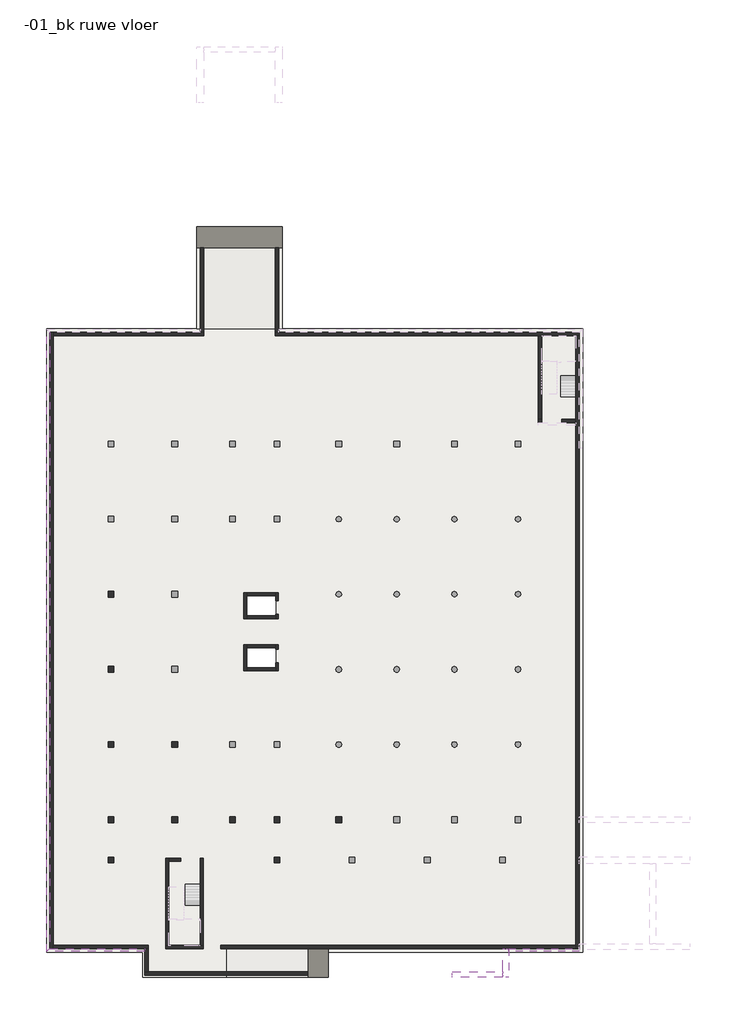
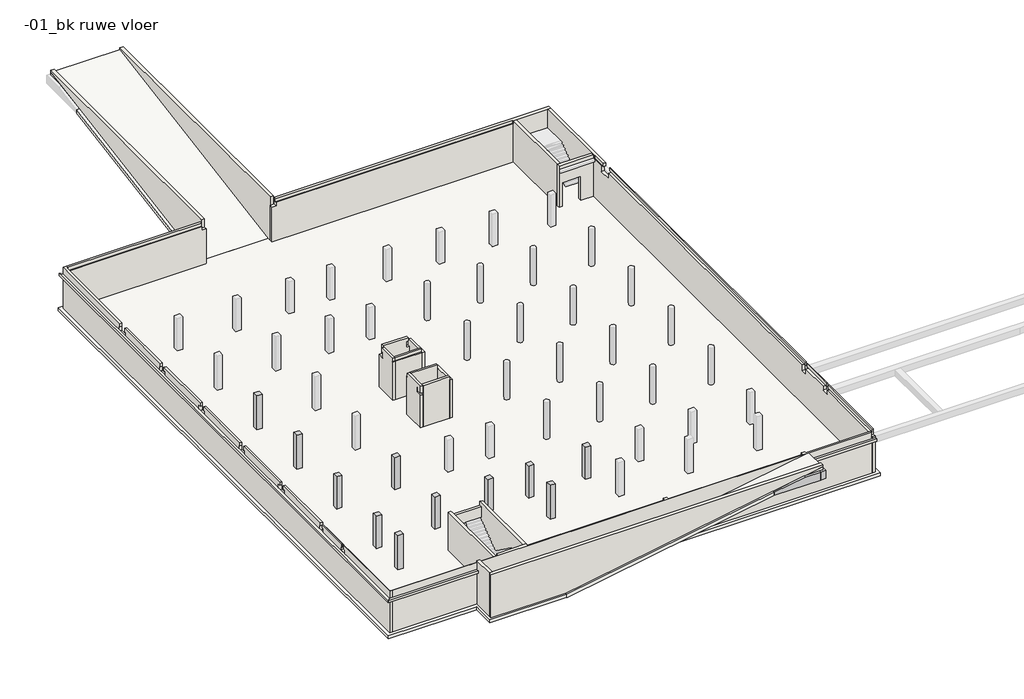
# One storey, part 1 of 2: 25 walls, 12 footings, 11 columns, 3 slabs, 2 beams.
"""IFC4 building model written with IfcOpenShell, lengths in millimetres."""

from ifc_helpers import new_model, si_unit, frame, origin, place, context, project, spatial, polyline, outline, extrude, faceted_brep, element, save

model = new_model("IFC4")

# Units and contexts
model_context = context("Model", 3, world=origin())
ifc_project = project(units=[si_unit("LENGTHUNIT", "METRE", prefix="MILLI")], contexts=[model_context])

# Site, building, storey
site = spatial("IfcSite", under=ifc_project)
building = spatial("IfcBuilding", under=site)
storey = spatial("IfcBuildingStorey", under=building, Name="-01_bk ruwe vloer", Elevation=-4200.0)

# Beams
placement = place(None, origin())
element("IfcBeam", 1, ObjectType="NLRS_16_SF_LIB_funderingsbalk beton ihwg-CWV-MMBC-SRP_gen_rsf : funderingsbalk beton ihwg_gen__bxh 500x800", at=placement, inside=storey, context=model_context, shape_type="Brep", body=[
    faceted_brep([(45545.0, -2650.0, -370.0), (46045.0, -2650.0, -370.0), (46045.0, -150.0, -370.0), (45845.0, -150.0, -370.0), (45845.0, -2450.0, -370.0), (45545.0, -2450.0, -370.0), (46045.0, -2650.0, -1170.0), (46045.0, -150.0, -1170.0), (45545.0, -2650.0, -1170.0), (45545.0, -2150.0, -1170.0), (45545.0, -150.0, -1170.0), (45545.0, -2450.0, -425.486389), (45545.0, -2150.0, -425.486389), (45545.0, -150.0, -425.486389), (45845.0, -150.0, -374.3303196), (45845.0, -2450.0, -374.3303196)], [[[0, 1, 2, 3, 4, 5]], [[1, 6, 7, 2]], [[6, 8, 9, 10, 7]], [[8, 0, 5, 11, 12, 13, 10, 9]], [[1, 0, 8, 6]], [[2, 7, 10, 13, 14, 3]], [[15, 14, 13, 12, 11]], [[14, 15, 4, 3]], [[15, 11, 5, 4]]]),
])
element("IfcBeam", 2, ObjectType="NLRS_16_SF_LIB_funderingsbalk beton ihwg-CWV-MMBC-SRP_gen_rsf : funderingsbalk beton ihwg_gen__bxh 500x800", at=placement, inside=storey, context=model_context, shape_type="Brep", body=[
    faceted_brep([(41178.8693319, -2650.0, -1170.0), (41178.8693319, -2650.0, -865.6696804), (41178.8693319, -2450.0, -865.6696804), (41178.8693319, -2450.0, -1170.0), (44085.6779661, -2650.0, -370.0), (45545.0, -2650.0, -370.0), (45545.0, -2450.0, -370.0), (44085.6779661, -2450.0, -370.0), (45545.0, -2650.0, -1170.0), (45545.0, -2150.0, -1170.0), (41178.8693319, -2150.0, -1170.0), (45545.0, -2150.0, -425.486389), (45545.0, -2450.0, -425.486389)], [[[0, 1, 2, 3]], [[4, 5, 6, 7]], [[1, 0, 8, 5, 4]], [[9, 8, 0, 3, 10]], [[9, 10, 11]], [[8, 9, 11, 12, 6, 5]], [[1, 4, 7, 2]], [[3, 12, 11, 10]], [[12, 3, 2, 7, 6]]]),
])

# Columns
element("IfcColumn", 3, ObjectType="NLRS_28_SCO_TLB_vierkante kolom beton prefab-BCPG-MMBPC-SRP_gen_rsf : kolom vierkant beton prefab_gen__bxh 500x500", at=placement, inside=storey, context=model_context, shape_type="SweptSolid", body=[
    extrude(outline(polyline([(26250.0, 7750.0), (26250.0, 7250.0), (25750.0, 7250.0), (25750.0, 7750.0), (26250.0, 7750.0)])), frame((0.0, 0.0, -4170.0), z_axis=(0.0, 0.0, 1.0), x_axis=(1.0, 0.0, 0.0)), (0.0, 0.0, 1.0), 3400.0),
])
element("IfcColumn", 4, ObjectType="NLRS_28_SCO_TLB_vierkante kolom beton prefab-BCPG-MMBPC-SRP_gen_rsf : kolom vierkant beton prefab_gen__bxh 500x500", at=placement, inside=storey, context=model_context, shape_type="SweptSolid", body=[
    extrude(outline(polyline([(31600.0, 11250.0), (31600.0, 10750.0), (31100.0, 10750.0), (31100.0, 11250.0), (31600.0, 11250.0)])), frame((0.0, 0.0, -4170.0), z_axis=(0.0, 0.0, 1.0), x_axis=(1.0, 0.0, 0.0)), (0.0, 0.0, 1.0), 3200.0),
])
element("IfcColumn", 5, ObjectType="NLRS_28_SCO_TLB_vierkante kolom beton prefab-BCPG-MMBPC-SRP_gen_rsf : kolom vierkant beton prefab_gen__bxh 500x500", at=placement, inside=storey, context=model_context, shape_type="SweptSolid", body=[
    extrude(outline(polyline([(26250.0, 11250.0), (26250.0, 10750.0), (25750.0, 10750.0), (25750.0, 11250.0), (26250.0, 11250.0)])), frame((0.0, 0.0, -4170.0), z_axis=(0.0, 0.0, 1.0), x_axis=(1.0, 0.0, 0.0)), (0.0, 0.0, 1.0), 3200.0),
])
element("IfcColumn", 6, ObjectType="NLRS_28_SCO_TLB_vierkante kolom beton prefab-BCPG-MMBPC-SRP_gen_rsf : kolom vierkant beton prefab_gen__bxh 500x500", at=placement, inside=storey, context=model_context, shape_type="SweptSolid", body=[
    extrude(outline(polyline([(17400.0, 11250.0), (17400.0, 10750.0), (16900.0, 10750.0), (16900.0, 11250.0), (17400.0, 11250.0)])), frame((0.0, 0.0, -4170.0), z_axis=(0.0, 0.0, 1.0), x_axis=(1.0, 0.0, 0.0)), (0.0, 0.0, 1.0), 3200.0),
])
element("IfcColumn", 7, ObjectType="NLRS_28_SCO_TLB_vierkante kolom beton prefab-BCPG-MMBPC-SRP_gen_rsf : kolom vierkant beton prefab_gen__bxh 500x500", at=placement, inside=storey, context=model_context, shape_type="SweptSolid", body=[
    extrude(outline(polyline([(17400.0, 17750.0), (17400.0, 17250.0), (16900.0, 17250.0), (16900.0, 17750.0), (17400.0, 17750.0)])), frame((0.0, 0.0, -4170.0), z_axis=(0.0, 0.0, 1.0), x_axis=(1.0, 0.0, 0.0)), (0.0, 0.0, 1.0), 3200.0),
])
element("IfcColumn", 8, ObjectType="NLRS_28_SCO_TLB_vierkante kolom beton prefab-BCPG-MMBPC-SRP_gen_rsf : kolom vierkant beton prefab_gen__bxh 500x500", at=placement, inside=storey, context=model_context, shape_type="SweptSolid", body=[
    extrude(outline(polyline([(11900.0, 11250.0), (11900.0, 10750.0), (11400.0, 10750.0), (11400.0, 11250.0), (11900.0, 11250.0)])), frame((0.0, 0.0, -4170.0), z_axis=(0.0, 0.0, 1.0), x_axis=(1.0, 0.0, 0.0)), (0.0, 0.0, 1.0), 3200.0),
])
element("IfcColumn", 9, ObjectType="NLRS_28_SCO_TLB_vierkante kolom beton prefab-BCPG-MMBPC-SRP_gen_rsf : kolom vierkant beton prefab_gen__bxh 500x500", at=placement, inside=storey, context=model_context, shape_type="SweptSolid", body=[
    extrude(outline(polyline([(11900.0, 17750.0), (11900.0, 17250.0), (11400.0, 17250.0), (11400.0, 17750.0), (11900.0, 17750.0)])), frame((0.0, 0.0, -4170.0), z_axis=(0.0, 0.0, 1.0), x_axis=(1.0, 0.0, 0.0)), (0.0, 0.0, 1.0), 3200.0),
])
element("IfcColumn", 10, ObjectType="NLRS_28_SCO_TLB_vierkante kolom beton prefab-BCPG-MMBPC-SRP_gen_rsf : kolom vierkant beton prefab_gen__bxh 500x500", at=placement, inside=storey, context=model_context, shape_type="SweptSolid", body=[
    extrude(outline(polyline([(11900.0, 24250.0), (11900.0, 23750.0), (11400.0, 23750.0), (11400.0, 24250.0), (11900.0, 24250.0)])), frame((0.0, 0.0, -4170.0), z_axis=(0.0, 0.0, 1.0), x_axis=(1.0, 0.0, 0.0)), (0.0, 0.0, 1.0), 3400.0),
])
element("IfcColumn", 11, ObjectType="NLRS_28_SCO_TLB_vierkante kolom beton prefab-BCPG-MMBPC-SRP_gen_rsf : kolom vierkant beton prefab_gen__bxh 500x500", at=placement, inside=storey, context=model_context, shape_type="SweptSolid", body=[
    extrude(outline(polyline([(11900.0, 30750.0), (11900.0, 30250.0), (11400.0, 30250.0), (11400.0, 30750.0), (11900.0, 30750.0)])), frame((0.0, 0.0, -4170.0), z_axis=(0.0, 0.0, 1.0), x_axis=(1.0, 0.0, 0.0)), (0.0, 0.0, 1.0), 3400.0),
])
element("IfcColumn", 12, ObjectType="NLRS_28_SCO_TLB_vierkante kolom beton prefab-BCPG-MMBPC-SRP_gen_rsf : kolom vierkant beton prefab_gen__bxh 500x500", at=placement, inside=storey, context=model_context, shape_type="SweptSolid", body=[
    extrude(outline(polyline([(11900.0, 7750.0), (11900.0, 7250.0), (11400.0, 7250.0), (11400.0, 7750.0), (11900.0, 7750.0)])), frame((0.0, 0.0, -4170.0), z_axis=(0.0, 0.0, 1.0), x_axis=(1.0, 0.0, 0.0)), (0.0, 0.0, 1.0), 3400.0),
])
element("IfcColumn", 13, ObjectType="NLRS_28_SCO_TLB_vierkante kolom beton prefab-BCPG-MMBPC-SRP_gen_rsf : kolom vierkant beton prefab_gen__bxh 500x500", at=placement, inside=storey, context=model_context, shape_type="SweptSolid", body=[
    extrude(outline(polyline([(22400.0, 11250.0), (22400.0, 10750.0), (21900.0, 10750.0), (21900.0, 11250.0), (22400.0, 11250.0)])), frame((0.0, 0.0, -4170.0), z_axis=(0.0, 0.0, 1.0), x_axis=(1.0, 0.0, 0.0)), (0.0, 0.0, 1.0), 3200.0),
])

# Footings
element("IfcFooting", 14, ObjectType="NLRS_16_SFO_LB_funderingspoer meerpaals beton ihwg-MMBC-SH_gen_rsf : funderingspoer beton ihwg_gen__4-paals bxlxh 1800x1800x1200", at=placement, inside=storey, context=model_context, shape_type="SweptSolid", body=[
    extrude(outline(polyline([(16250.0, 16600.0), (16250.0, 18400.0), (18050.0, 18400.0), (18050.0, 16600.0), (16250.0, 16600.0)])), frame((0.0, 0.0, -5400.0), z_axis=(0.0, 0.0, 1.0), x_axis=(1.0, 0.0, 0.0)), (0.0, 0.0, 1.0), 900.0),
])
element("IfcFooting", 15, ObjectType="NLRS_16_SFO_LB_funderingspoer meerpaals beton ihwg-MMBC-SH_gen_rsf : funderingspoer beton ihwg_gen__3-paals bxlxh 1800x1800x1200", at=placement, inside=storey, context=model_context, shape_type="SweptSolid", body=[
    extrude(outline(polyline([(18050.0, 12075.0), (18050.0, 10275.0), (16250.0, 10275.0), (16250.0, 12075.0), (18050.0, 12075.0)])), frame((0.0, 0.0, -5400.0), z_axis=(0.0, 0.0, 1.0), x_axis=(1.0, 0.0, 0.0)), (0.0, 0.0, 1.0), 900.0),
])
element("IfcFooting", 16, ObjectType="NLRS_16_SFO_LB_funderingspoer meerpaals beton ihwg-MMBC-SH_gen_rsf : funderingspoer beton ihwg_gen__2-paals bxlxh 700x1800x1200", at=placement, inside=storey, context=model_context, shape_type="SweptSolid", body=[
    extrude(outline(polyline([(11300.0, 31400.0), (12000.0, 31400.0), (12000.0, 29600.0), (11300.0, 29600.0), (11300.0, 31400.0)])), frame((0.0, 0.0, -5400.0), z_axis=(0.0, 0.0, 1.0), x_axis=(1.0, 0.0, 0.0)), (0.0, 0.0, 1.0), 900.0),
])
element("IfcFooting", 17, ObjectType="NLRS_16_SFO_LB_funderingspoer meerpaals beton ihwg-MMBC-SH_gen_rsf : funderingspoer beton ihwg_gen__2-paals bxlxh 700x1800x1200", at=placement, inside=storey, context=model_context, shape_type="SweptSolid", body=[
    extrude(outline(polyline([(11300.0, 24900.0), (12000.0, 24900.0), (12000.0, 23100.0), (11300.0, 23100.0), (11300.0, 24900.0)])), frame((0.0, 0.0, -5400.0), z_axis=(0.0, 0.0, 1.0), x_axis=(1.0, 0.0, 0.0)), (0.0, 0.0, 1.0), 900.0),
])
element("IfcFooting", 18, ObjectType="NLRS_16_SFO_LB_funderingspoer meerpaals beton ihwg-MMBC-SH_gen_rsf : funderingspoer beton ihwg_gen__2-paals bxlxh 700x1800x1200", at=placement, inside=storey, context=model_context, shape_type="SweptSolid", body=[
    extrude(outline(polyline([(11300.0, 18400.0), (12000.0, 18400.0), (12000.0, 16600.0), (11300.0, 16600.0), (11300.0, 18400.0)])), frame((0.0, 0.0, -5400.0), z_axis=(0.0, 0.0, 1.0), x_axis=(1.0, 0.0, 0.0)), (0.0, 0.0, 1.0), 900.0),
])
element("IfcFooting", 19, ObjectType="NLRS_16_SFO_LB_funderingspoer meerpaals beton ihwg-MMBC-SH_gen_rsf : funderingspoer beton ihwg_gen__1-paals bxlxh 700x700x500", at=placement, inside=storey, context=model_context, shape_type="SweptSolid", body=[
    extrude(outline(polyline([(11300.0, 11350.0), (12000.0, 11350.0), (12000.0, 10650.0), (11300.0, 10650.0), (11300.0, 11350.0)])), frame((0.0, 0.0, -4700.0), z_axis=(0.0, 0.0, 1.0), x_axis=(1.0, 0.0, 0.0)), (0.0, 0.0, 1.0), 200.0),
])
element("IfcFooting", 20, ObjectType="NLRS_16_SFO_LB_funderingspoer meerpaals beton ihwg-MMBC-SH_gen_rsf : funderingspoer beton ihwg_gen__1-paals bxlxh 700x700x500", at=placement, inside=storey, context=model_context, shape_type="SweptSolid", body=[
    extrude(outline(polyline([(11300.0, 7850.0), (12000.0, 7850.0), (12000.0, 7150.0), (11300.0, 7150.0), (11300.0, 7850.0)])), frame((0.0, 0.0, -4700.0), z_axis=(0.0, 0.0, 1.0), x_axis=(1.0, 0.0, 0.0)), (0.0, 0.0, 1.0), 200.0),
])
element("IfcFooting", 21, ObjectType="NLRS_16_SFO_LB_funderingspoer meerpaals beton ihwg-MMBC-SH_gen_rsf : funderingspoer beton ihwg_gen__1-paals bxlxh 700x700x500", at=placement, inside=storey, context=model_context, shape_type="SweptSolid", body=[
    extrude(outline(polyline([(21800.0, 11350.0), (22500.0, 11350.0), (22500.0, 10650.0), (21800.0, 10650.0), (21800.0, 11350.0)])), frame((0.0, 0.0, -4700.0), z_axis=(0.0, 0.0, 1.0), x_axis=(1.0, 0.0, 0.0)), (0.0, 0.0, 1.0), 200.0),
])
element("IfcFooting", 22, ObjectType="NLRS_16_SFO_LB_funderingspoer meerpaals beton ihwg-MMBC-SH_gen_rsf : funderingspoer beton ihwg_gen__2-paals bxlxh 700x1800x1200", at=placement, inside=storey, context=model_context, shape_type="SweptSolid", body=[
    extrude(outline(polyline([(31000.0, 11900.0), (31700.0, 11900.0), (31700.0, 10100.0), (31000.0, 10100.0), (31000.0, 11900.0)])), frame((0.0, 0.0, -5400.0), z_axis=(0.0, 0.0, 1.0), x_axis=(1.0, 0.0, 0.0)), (0.0, 0.0, 1.0), 900.0),
])
element("IfcFooting", 23, ObjectType="NLRS_16_SFO_LB_funderingspoer meerpaals beton ihwg-MMBC-SH_gen_rsf : funderingspoer beton ihwg_gen__4-paals bxlxh 1800x1800x1200", at=placement, inside=storey, context=model_context, shape_type="SweptSolid", body=[
    extrude(outline(polyline([(25100.0, 6600.0), (25100.0, 8400.0), (26900.0, 8400.0), (26900.0, 6600.0), (25100.0, 6600.0)])), frame((0.0, 0.0, -5400.0), z_axis=(0.0, 0.0, 1.0), x_axis=(1.0, 0.0, 0.0)), (0.0, 0.0, 1.0), 900.0),
])
element("IfcFooting", 24, ObjectType="NLRS_16_SFO_LB_funderingspoer meerpaals beton ihwg-MMBC-SH_gen_rsf : funderingspoer beton ihwg_gen__trap bxlxh 3800x9300x1200", at=placement, inside=storey, context=model_context, shape_type="SweptSolid", body=[
    extrude(outline(polyline([(19900.0, -900.0), (16100.0, -900.0), (16100.0, 8400.0), (19900.0, 8400.0), (19900.0, -900.0)])), frame((0.0, 0.0, -5400.0), z_axis=(0.0, 0.0, 1.0), x_axis=(1.0, 0.0, 0.0)), (0.0, 0.0, 1.0), 900.0),
])
element("IfcFooting", 25, ObjectType="NLRS_16_SFO_LB_funderingspoer meerpaals beton ihwg-MMBC-SH_gen_rsf : funderingspoer beton ihwg_gen__3-paals bxlxh 1800x1800x1200", at=placement, inside=storey, context=model_context, shape_type="SweptSolid", body=[
    extrude(outline(polyline([(26900.0, 12075.0), (26900.0, 10275.0), (25100.0, 10275.0), (25100.0, 12075.0), (26900.0, 12075.0)])), frame((0.0, 0.0, -5400.0), z_axis=(0.0, 0.0, 1.0), x_axis=(1.0, 0.0, 0.0)), (0.0, 0.0, 1.0), 900.0),
])

# Slabs
element("IfcSlab", 26, ObjectType="NLRS_13_FL_beton ihwg 300_gen_rsf", at=placement, inside=storey, context=model_context, shape_type="Brep", body=[
    faceted_brep([(6070.0, 53450.0, -4500.0), (48305.0, 53450.0, -4500.0), (52450.0, 53450.0, -4500.0), (52450.0, 45050.0, -4500.0), (52450.0, -450.0, -4500.0), (21650.3947557, -450.0, -4500.0), (21625.0, -450.0, -4500.0), (21625.0, -2650.0, -4500.0), (14375.0, -2650.0, -4500.0), (14375.0, -450.0, -4500.0), (6070.0, -450.0, -4500.0), (25875.0, 30375.0, -4500.0), (23375.0, 30375.0, -4500.0), (23375.0, 28625.0, -4500.0), (25875.0, 28625.0, -4500.0), (25875.0, 25875.0, -4500.0), (23375.0, 25875.0, -4500.0), (23375.0, 24125.0, -4500.0), (25875.0, 24125.0, -4500.0), (6070.0, 53450.0, -4200.0), (6070.0, -450.0, -4200.0), (14375.0, -450.0, -4200.0), (14375.0, -2650.0, -4200.0), (21625.0, -2650.0, -4200.0), (21625.0, -450.0, -4200.0), (23409.7167896, -450.0, -4200.0), (52450.0, -450.0, -4200.0), (52450.0, 53450.0, -4200.0), (25875.0, 25875.0, -4200.0), (25875.0, 25752.0, -4200.0), (25875.0, 24552.0, -4200.0), (25875.0, 24125.0, -4200.0), (23375.0, 24125.0, -4200.0), (23375.0, 25875.0, -4200.0), (25875.0, 30375.0, -4200.0), (25875.0, 29948.0, -4200.0), (25875.0, 28748.0, -4200.0), (25875.0, 28625.0, -4200.0), (23375.0, 28625.0, -4200.0), (23375.0, 30375.0, -4200.0)], [[[0, 1, 2, 3, 4, 5, 6, 7, 8, 9, 10], [11, 12, 13, 14], [15, 16, 17, 18]], [[19, 20, 21, 22, 23, 24, 25, 26, 27], [28, 29, 30, 31, 32, 33], [34, 35, 36, 37, 38, 39]], [[4, 3, 2, 27, 26]], [[6, 5, 4, 26, 25, 24]], [[0, 10, 20, 19]], [[7, 6, 24, 23]], [[8, 7, 23, 22]], [[9, 8, 22, 21]], [[10, 9, 21, 20]], [[2, 1, 0, 19, 27]], [[12, 11, 34, 39]], [[13, 12, 39, 38]], [[14, 13, 38, 37]], [[11, 14, 37, 36, 35, 34]], [[16, 15, 28, 33]], [[17, 16, 33, 32]], [[18, 17, 32, 31]], [[15, 18, 31, 30, 29, 28]]]),
])
element("IfcSlab", 27, ObjectType="NLRS_13_FL_beton ihwg 300_gen_rsf", at=placement, inside=storey, context=model_context, shape_type="Brep", body=[
    faceted_brep([(19050.0, 53450.0, -4504.3303196), (19050.0, 73003.8693319, -1170.0), (19350.0, 73003.8693319, -1170.0), (19350.0, 77670.0, -374.3303196), (19650.0, 77670.0, -374.3303196), (25850.0, 77670.0, -374.3303196), (26150.0, 77670.0, -374.3303196), (26150.0, 73003.8693319, -1170.0), (26450.0, 73003.8693319, -1170.0), (26450.0, 53450.0, -4504.3303196), (19050.0, 53450.0, -4200.0), (26450.0, 53450.0, -4200.0), (26450.0, 73003.8693319, -865.6696804), (26150.0, 73003.8693319, -865.6696804), (26150.0, 75910.6779661, -370.0), (26150.0, 77670.0, -70.0), (25850.0, 77670.0, -70.0), (19650.0, 77670.0, -70.0), (19350.0, 77670.0, -70.0), (19350.0, 75910.6779661, -370.0), (19350.0, 73003.8693319, -865.6696804), (19050.0, 73003.8693319, -865.6696804), (19350.0, 77670.0, -370.0), (26150.0, 77670.0, -370.0)], [[[0, 1, 2, 3, 4, 5, 6, 7, 8, 9]], [[10, 11, 12, 13, 14, 15, 16, 17, 18, 19, 20, 21]], [[1, 0, 10, 21]], [[6, 5, 4, 3, 22, 18, 17, 16, 15, 23]], [[9, 8, 12, 11]], [[0, 9, 11, 10]], [[2, 1, 21, 20]], [[3, 2, 20, 19, 18, 22]], [[7, 6, 23, 15, 14, 13]], [[8, 7, 13, 12]]]),
])
element("IfcSlab", 28, ObjectType="NLRS_13_FL_beton ihwg 300_gen_rsf", at=placement, inside=storey, context=model_context, shape_type="Brep", body=[
    faceted_brep([(45845.0, -150.0, -374.3303196), (45845.0, -2450.0, -374.3303196), (45545.0, -2450.0, -425.486389), (41178.8693319, -2450.0, -1170.0), (41178.8693319, -2650.0, -1170.0), (21625.0, -2650.0, -4504.3303196), (21625.0, -150.0, -4504.3303196), (21650.3947557, -150.0, -4500.0), (21650.3947557, -450.0, -4500.0), (23409.7167896, -450.0, -4200.0), (23409.7167896, -150.0, -4200.0), (45545.0, -150.0, -425.486389), (45845.0, -2450.0, -70.0), (45845.0, -2150.0, -70.0), (45845.0, -150.0, -70.0), (21625.0, -150.0, -4200.0), (21625.0, -450.0, -4200.0), (21625.0, -2650.0, -4200.0), (41178.8693319, -2650.0, -865.6696804), (41178.8693319, -2450.0, -865.6696804), (44085.6779661, -2450.0, -370.0), (45845.0, -150.0, -370.0), (45845.0, -2450.0, -370.0), (21625.0, -2650.0, -4500.0), (21625.0, -450.0, -4500.0), (21625.0, -150.0, -4500.0)], [[[0, 1, 2, 3, 4, 5, 6, 7, 8, 9, 10, 11]], [[12, 13, 14, 15, 16, 17, 18, 19, 20]], [[1, 0, 21, 14, 13, 12, 22]], [[5, 4, 18, 17, 23]], [[6, 5, 23, 17, 16, 24, 25]], [[15, 14, 21, 0, 11, 10]], [[7, 6, 25]], [[24, 8, 7, 25]], [[9, 16, 15, 10]], [[8, 24, 16, 9]], [[3, 2, 1, 22, 12, 20, 19]], [[4, 3, 19, 18]]]),
])

# Walls
element("IfcWall", 29, ObjectType="NLRS_16_WA_hollewand 300_gen_rsf", at=placement, inside=storey, context=model_context, shape_type="Brep", body=[
    faceted_brep([(6650.0, -150.0, -4200.0), (6650.0, 150.0, -4200.0), (6650.0, 52850.0, -4200.0), (6650.0, 53150.0, -4200.0), (6650.0, 53150.0, -70.0), (6650.0, 52950.0, -70.0), (6650.0, 52950.0, -390.0), (6650.0, 52850.0, -390.0), (6650.0, 44100.0, -390.0), (6650.0, 44100.0, -970.0), (6650.0, 42900.0, -970.0), (6650.0, 42900.0, -390.0), (6650.0, 37500.0, -390.0), (6650.0, 37500.0, -970.0), (6650.0, 36500.0, -970.0), (6650.0, 36500.0, -390.0), (6650.0, 31000.0, -390.0), (6650.0, 31000.0, -970.0), (6650.0, 30000.0, -970.0), (6650.0, 30000.0, -390.0), (6650.0, 24500.0, -390.0), (6650.0, 24500.0, -970.0), (6650.0, 23500.0, -970.0), (6650.0, 23500.0, -390.0), (6650.0, 18000.0, -390.0), (6650.0, 18000.0, -970.0), (6650.0, 17000.0, -970.0), (6650.0, 17000.0, -390.0), (6650.0, 11350.0, -390.0), (6650.0, 11350.0, -970.0), (6650.0, 10650.0, -970.0), (6650.0, 10650.0, -390.0), (6650.0, 7850.0, -390.0), (6650.0, 7850.0, -770.0), (6650.0, 7150.0, -770.0), (6650.0, 7150.0, -390.0), (6650.0, 150.0, -390.0), (6650.0, -90.0, -390.0), (6650.0, -90.0, -70.0), (6650.0, -150.0, -70.0), (6350.0, 53150.0, -4200.0), (6350.0, -150.0, -4200.0), (6350.0, -150.0, -70.0), (6350.0, 7350.0, -70.0), (6350.0, 7350.0, -390.0), (6350.0, 7150.0, -390.0), (6350.0, 7150.0, -770.0), (6350.0, 7850.0, -770.0), (6350.0, 7850.0, -390.0), (6350.0, 7650.0, -390.0), (6350.0, 7650.0, -70.0), (6350.0, 10850.0, -70.0), (6350.0, 10850.0, -390.0), (6350.0, 10650.0, -390.0), (6350.0, 10650.0, -970.0), (6350.0, 11350.0, -970.0), (6350.0, 11350.0, -390.0), (6350.0, 11150.0, -390.0), (6350.0, 11150.0, -70.0), (6350.0, 17200.0, -70.0), (6350.0, 17200.0, -390.0), (6350.0, 17000.0, -390.0), (6350.0, 17000.0, -970.0), (6350.0, 18000.0, -970.0), (6350.0, 18000.0, -390.0), (6350.0, 17800.0, -390.0), (6350.0, 17800.0, -70.0), (6350.0, 23700.0, -70.0), (6350.0, 23700.0, -390.0), (6350.0, 23500.0, -390.0), (6350.0, 23500.0, -970.0), (6350.0, 24500.0, -970.0), (6350.0, 24500.0, -390.0), (6350.0, 24300.0, -390.0), (6350.0, 24300.0, -70.0), (6350.0, 30200.0, -70.0), (6350.0, 30200.0, -390.0), (6350.0, 30000.0, -390.0), (6350.0, 30000.0, -970.0), (6350.0, 31000.0, -970.0), (6350.0, 31000.0, -390.0), (6350.0, 30800.0, -390.0), (6350.0, 30800.0, -70.0), (6350.0, 36700.0, -70.0), (6350.0, 36700.0, -390.0), (6350.0, 36500.0, -390.0), (6350.0, 36500.0, -970.0), (6350.0, 37500.0, -970.0), (6350.0, 37500.0, -390.0), (6350.0, 37300.0, -390.0), (6350.0, 37300.0, -70.0), (6350.0, 43100.0, -70.0), (6350.0, 43100.0, -390.0), (6350.0, 42900.0, -390.0), (6350.0, 42900.0, -970.0), (6350.0, 44100.0, -970.0), (6350.0, 44100.0, -390.0), (6350.0, 43900.0, -390.0), (6350.0, 43900.0, -70.0), (6350.0, 53150.0, -70.0), (6410.0, -90.0, -70.0), (6410.0, 7350.0, -70.0), (6410.0, 7650.0, -70.0), (6410.0, 10850.0, -70.0), (6550.0, 17800.0, -70.0), (6550.0, 23700.0, -70.0), (6550.0, 24300.0, -70.0), (6550.0, 30200.0, -70.0), (6550.0, 30800.0, -70.0), (6550.0, 36700.0, -70.0), (6550.0, 37300.0, -70.0), (6550.0, 43100.0, -70.0), (6550.0, 43900.0, -70.0), (6550.0, 52950.0, -70.0), (6550.0, 11150.0, -70.0), (6550.0, 17200.0, -70.0), (6410.0, -90.0, -390.0), (6410.0, 7150.0, -390.0), (6410.0, 7350.0, -390.0), (6550.0, 17200.0, -390.0), (6550.0, 17800.0, -390.0), (6550.0, 23700.0, -390.0), (6550.0, 24300.0, -390.0), (6550.0, 30200.0, -390.0), (6550.0, 30800.0, -390.0), (6550.0, 36700.0, -390.0), (6550.0, 37300.0, -390.0), (6550.0, 43100.0, -390.0), (6550.0, 42900.0, -390.0), (6550.0, 44100.0, -390.0), (6550.0, 43900.0, -390.0), (6550.0, 36500.0, -390.0), (6550.0, 37500.0, -390.0), (6550.0, 30000.0, -390.0), (6550.0, 31000.0, -390.0), (6550.0, 23500.0, -390.0), (6550.0, 24500.0, -390.0), (6550.0, 17000.0, -390.0), (6550.0, 18000.0, -390.0), (6410.0, 10650.0, -390.0), (6410.0, 7850.0, -390.0), (6410.0, 7650.0, -390.0), (6410.0, 10850.0, -390.0), (6550.0, 11350.0, -390.0), (6550.0, 11150.0, -390.0), (6550.0, 52950.0, -390.0)], [[[0, 1, 2, 3, 4, 5, 6, 7, 8, 9, 10, 11, 12, 13, 14, 15, 16, 17, 18, 19, 20, 21, 22, 23, 24, 25, 26, 27, 28, 29, 30, 31, 32, 33, 34, 35, 36, 37, 38, 39]], [[40, 41, 42, 43, 44, 45, 46, 47, 48, 49, 50, 51, 52, 53, 54, 55, 56, 57, 58, 59, 60, 61, 62, 63, 64, 65, 66, 67, 68, 69, 70, 71, 72, 73, 74, 75, 76, 77, 78, 79, 80, 81, 82, 83, 84, 85, 86, 87, 88, 89, 90, 91, 92, 93, 94, 95, 96, 97, 98, 99]], [[3, 2, 1, 0, 41, 40]], [[42, 39, 38, 100, 101, 43]], [[102, 103, 51, 50]], [[67, 66, 104, 105]], [[75, 74, 106, 107]], [[83, 82, 108, 109]], [[91, 90, 110, 111]], [[99, 98, 112, 113, 5, 4]], [[59, 58, 114, 115]], [[0, 39, 42, 41]], [[116, 37, 36, 35, 117]], [[116, 100, 38, 37]], [[100, 116, 117, 118, 101]], [[59, 115, 119, 60]], [[104, 66, 65, 120]], [[67, 105, 121, 68]], [[106, 74, 73, 122]], [[75, 107, 123, 76]], [[108, 82, 81, 124]], [[83, 109, 125, 84]], [[110, 90, 89, 126]], [[92, 91, 111, 127]], [[93, 92, 127, 128]], [[10, 94, 93, 128, 11]], [[94, 10, 9, 95]], [[95, 9, 8, 129, 96]], [[97, 96, 129, 130]], [[98, 97, 130, 112]], [[14, 86, 85, 131, 15]], [[86, 14, 13, 87]], [[87, 13, 12, 132, 88]], [[89, 88, 132, 126]], [[85, 84, 125, 131]], [[19, 18, 78, 77, 133]], [[17, 79, 78, 18]], [[79, 17, 16, 134, 80]], [[81, 80, 134, 124]], [[77, 76, 123, 133]], [[22, 70, 69, 135, 23]], [[70, 22, 21, 71]], [[71, 21, 20, 136, 72]], [[73, 72, 136, 122]], [[69, 68, 121, 135]], [[26, 62, 61, 137, 27]], [[62, 26, 25, 63]], [[63, 25, 24, 138, 64]], [[65, 64, 138, 120]], [[61, 60, 119, 137]], [[31, 139, 140, 32]], [[103, 102, 141, 140, 139, 142]], [[142, 52, 51, 103]], [[52, 142, 139, 53]], [[53, 139, 31, 30, 54]], [[54, 30, 29, 55]], [[55, 29, 28, 143, 56]], [[57, 56, 143, 144]], [[58, 57, 144, 114]], [[145, 129, 8, 7, 6]], [[145, 113, 112, 130, 129]], [[12, 11, 128, 132]], [[111, 110, 126, 132, 128, 127]], [[16, 15, 131, 134]], [[109, 108, 124, 134, 131, 125]], [[20, 19, 133, 136]], [[107, 106, 122, 136, 133, 123]], [[24, 23, 135, 138]], [[105, 104, 120, 138, 135, 121]], [[28, 27, 137, 143]], [[115, 114, 144, 143, 137, 119]], [[118, 44, 43, 101]], [[44, 118, 117, 45]], [[45, 117, 35, 34, 46]], [[46, 34, 33, 47]], [[140, 48, 47, 33, 32]], [[141, 49, 48, 140]], [[49, 141, 102, 50]], [[4, 3, 40, 99]], [[113, 145, 6, 5]]]),
])
element("IfcWall", 30, ObjectType="NLRS_16_WA_hollewand 300_gen_rsf", at=placement, inside=storey, context=model_context, shape_type="Brep", body=[
    faceted_brep([(6650.0, 52850.0, -4200.0), (19650.0, 52850.0, -4200.0), (19650.0, 52850.0, -720.0), (19250.0, 52850.0, -720.0), (19250.0, 52850.0, -390.0), (6650.0, 52850.0, -390.0), (19650.0, 53150.0, -4200.0), (6650.0, 53150.0, -4200.0), (6650.0, 53150.0, -70.0), (19250.0, 53150.0, -70.0), (19250.0, 53150.0, -720.0), (19650.0, 53150.0, -720.0), (6650.0, 52950.0, -70.0), (19250.0, 52950.0, -70.0), (19250.0, 52950.0, -390.0), (6650.0, 52950.0, -390.0)], [[[0, 1, 2, 3, 4, 5]], [[6, 7, 8, 9, 10, 11]], [[1, 0, 7, 6]], [[1, 6, 11, 2]], [[12, 13, 9, 8]], [[5, 4, 14, 15]], [[13, 12, 15, 14]], [[3, 10, 9, 13, 14, 4]], [[10, 3, 2, 11]], [[8, 7, 0, 5, 15, 12]]]),
])
element("IfcWall", 31, ObjectType="NLRS_16_WA_hollewand 300_gen_rsf", at=placement, inside=storey, context=model_context, shape_type="Brep", body=[
    faceted_brep([(25850.0, 52850.0, -4200.0), (51850.0, 52850.0, -4200.0), (52150.0, 52850.0, -4200.0), (52150.0, 52850.0, -70.0), (51850.0, 52850.0, -70.0), (48605.0, 52850.0, -70.0), (48605.0, 52850.0, -390.0), (26250.0, 52850.0, -390.0), (26250.0, 52850.0, -720.0), (25850.0, 52850.0, -720.0), (52150.0, 53150.0, -4200.0), (25850.0, 53150.0, -4200.0), (25850.0, 53150.0, -720.0), (26250.0, 53150.0, -720.0), (26250.0, 53150.0, -70.0), (52150.0, 53150.0, -70.0), (26250.0, 52950.0, -70.0), (48605.0, 52950.0, -70.0), (48605.0, 52950.0, -390.0), (26250.0, 52950.0, -390.0)], [[[0, 1, 2, 3, 4, 5, 6, 7, 8, 9]], [[10, 11, 12, 13, 14, 15]], [[2, 1, 0, 11, 10]], [[3, 15, 14, 16, 17, 5, 4]], [[11, 0, 9, 12]], [[3, 2, 10, 15]], [[6, 18, 19, 7]], [[18, 6, 5, 17]], [[19, 18, 17, 16]], [[13, 8, 7, 19, 16, 14]], [[8, 13, 12, 9]]]),
])
element("IfcWall", 32, ObjectType="NLRS_16_WA_hollewand 300_gen_rsf", at=placement, inside=storey, context=model_context, shape_type="Brep", body=[
    faceted_brep([(51850.0, 52850.0, -4200.0), (51850.0, 150.0, -4200.0), (51850.0, -150.0, -4200.0), (51850.0, -150.0, -590.0), (51850.0, 150.0, -590.0), (51850.0, 150.0, -390.0), (51850.0, 7150.0, -390.0), (51850.0, 7150.0, -770.0), (51850.0, 7850.0, -770.0), (51850.0, 7850.0, -390.0), (51850.0, 10650.0, -390.0), (51850.0, 10650.0, -970.0), (51850.0, 11350.0, -970.0), (51850.0, 11350.0, -390.0), (51850.0, 42900.0, -390.0), (51850.0, 42900.0, -970.0), (51850.0, 44100.0, -970.0), (51850.0, 44100.0, -390.0), (51850.0, 45270.0, -390.0), (51850.0, 45270.0, -70.0), (51850.0, 52850.0, -70.0), (52150.0, -150.0, -4200.0), (52150.0, 52850.0, -4200.0), (52150.0, 52850.0, -70.0), (52150.0, 43900.0, -70.0), (52150.0, 43900.0, -390.0), (52150.0, 44100.0, -390.0), (52150.0, 44100.0, -970.0), (52150.0, 42900.0, -970.0), (52150.0, 42900.0, -390.0), (52150.0, 43100.0, -390.0), (52150.0, 43100.0, -70.0), (52150.0, 11150.0, -70.0), (52150.0, 11150.0, -390.0), (52150.0, 11350.0, -390.0), (52150.0, 11350.0, -970.0), (52150.0, 10650.0, -970.0), (52150.0, 10650.0, -390.0), (52150.0, 10850.0, -390.0), (52150.0, 10850.0, -70.0), (52150.0, 7650.0, -70.0), (52150.0, 7650.0, -390.0), (52150.0, 7850.0, -390.0), (52150.0, 7850.0, -770.0), (52150.0, 7150.0, -770.0), (52150.0, 7150.0, -390.0), (52150.0, 7350.0, -390.0), (52150.0, 7350.0, -70.0), (52150.0, 150.0, -70.0), (52150.0, 150.0, -590.0), (52150.0, -150.0, -590.0), (51950.0, 45270.0, -70.0), (51950.0, 43900.0, -70.0), (52090.0, 10850.0, -70.0), (52090.0, 7650.0, -70.0), (52090.0, 43100.0, -70.0), (52090.0, 11150.0, -70.0), (52050.0, 7350.0, -70.0), (52050.0, 150.0, -70.0), (52090.0, 43100.0, -390.0), (52090.0, 42900.0, -390.0), (51950.0, 44100.0, -390.0), (51950.0, 43900.0, -390.0), (52090.0, 7850.0, -390.0), (52090.0, 10650.0, -390.0), (52090.0, 10850.0, -390.0), (52090.0, 7650.0, -390.0), (51950.0, 45270.0, -390.0), (52090.0, 11350.0, -390.0), (52090.0, 11150.0, -390.0), (52050.0, 7150.0, -390.0), (52050.0, 150.0, -390.0), (52050.0, 7350.0, -390.0)], [[[0, 1, 2, 3, 4, 5, 6, 7, 8, 9, 10, 11, 12, 13, 14, 15, 16, 17, 18, 19, 20]], [[21, 22, 23, 24, 25, 26, 27, 28, 29, 30, 31, 32, 33, 34, 35, 36, 37, 38, 39, 40, 41, 42, 43, 44, 45, 46, 47, 48, 49, 50]], [[2, 1, 0, 22, 21]], [[23, 20, 19, 51, 52, 24]], [[53, 54, 40, 39]], [[31, 55, 56, 32]], [[47, 57, 58, 48]], [[0, 20, 23, 22]], [[2, 21, 50, 3]], [[31, 30, 59, 55]], [[30, 29, 60, 59]], [[28, 15, 14, 60, 29]], [[15, 28, 27, 16]], [[16, 27, 26, 61, 17]], [[26, 25, 62, 61]], [[25, 24, 52, 62]], [[9, 63, 64, 10]], [[54, 53, 65, 64, 63, 66]], [[61, 67, 18, 17]], [[67, 61, 62, 52, 51]], [[60, 14, 13, 68]], [[56, 55, 59, 60, 68, 69]], [[67, 51, 19, 18]], [[70, 6, 5, 71]], [[57, 72, 70, 71, 58]], [[46, 72, 57, 47]], [[72, 46, 45, 70]], [[70, 45, 44, 7, 6]], [[7, 44, 43, 8]], [[42, 63, 9, 8, 43]], [[63, 42, 41, 66]], [[66, 41, 40, 54]], [[38, 65, 53, 39]], [[65, 38, 37, 64]], [[64, 37, 36, 11, 10]], [[11, 36, 35, 12]], [[34, 68, 13, 12, 35]], [[68, 34, 33, 69]], [[69, 33, 32, 56]], [[49, 4, 3, 50]], [[4, 49, 48, 58, 71, 5]]]),
])
element("IfcWall", 33, ObjectType="NLRS_16_WA_hollewand 300_gen_rsf", at=placement, inside=storey, context=model_context, shape_type="Brep", body=[
    faceted_brep([(6650.0, 150.0, -4200.0), (6650.0, 150.0, -390.0), (16625.0, 150.0, -390.0), (16625.0, 150.0, -70.0), (19375.0, 150.0, -70.0), (19375.0, 150.0, -390.0), (32350.0, 150.0, -390.0), (32350.0, 150.0, -70.0), (32650.0, 150.0, -70.0), (32650.0, 150.0, -390.0), (45350.0, 150.0, -390.0), (45350.0, 150.0, -70.0), (45650.0, 150.0, -70.0), (45650.0, 150.0, -390.0), (51750.0, 150.0, -390.0), (51750.0, 150.0, -590.0), (51850.0, 150.0, -590.0), (51850.0, 150.0, -4200.0), (21125.0, 150.0, -4200.0), (21125.0, 150.0, -1700.0), (19625.0, 150.0, -1700.0), (19625.0, 150.0, -4200.0), (16375.0, 150.0, -4200.0), (16375.0, 150.0, -1700.0), (14875.0, 150.0, -1700.0), (14875.0, 150.0, -4200.0), (6650.0, -150.0, -70.0), (6650.0, -150.0, -4200.0), (14575.0, -150.0, -4200.0), (14875.0, -150.0, -4200.0), (14875.0, -150.0, -1700.0), (16375.0, -150.0, -1700.0), (16375.0, -150.0, -4200.0), (19625.0, -150.0, -4200.0), (19625.0, -150.0, -1700.0), (21125.0, -150.0, -1700.0), (21125.0, -150.0, -4200.0), (51850.0, -150.0, -4200.0), (51850.0, -150.0, -590.0), (51750.0, -150.0, -590.0), (51750.0, -150.0, -70.0), (39200.0, -150.0, -70.0), (38800.0, -150.0, -70.0), (26200.0, -150.0, -70.0), (25800.0, -150.0, -70.0), (6650.0, -90.0, -70.0), (51750.0, -50.0, -70.0), (45650.0, -50.0, -70.0), (45350.0, -90.0, -70.0), (32650.0, -90.0, -70.0), (32350.0, -90.0, -70.0), (19375.0, -90.0, -70.0), (16625.0, -90.0, -70.0), (6650.0, -90.0, -390.0), (16625.0, -90.0, -390.0), (45650.0, -50.0, -390.0), (51750.0, -50.0, -390.0), (32650.0, -90.0, -390.0), (45350.0, -90.0, -390.0), (19375.0, -90.0, -390.0), (32350.0, -90.0, -390.0)], [[[0, 1, 2, 3, 4, 5, 6, 7, 8, 9, 10, 11, 12, 13, 14, 15, 16, 17, 18, 19, 20, 21, 22, 23, 24, 25]], [[26, 27, 28, 29, 30, 31, 32, 33, 34, 35, 36, 37, 38, 39, 40, 41, 42, 43, 44]], [[17, 37, 36, 18]], [[27, 0, 25, 29, 28]], [[32, 22, 21, 33]], [[45, 26, 44, 43, 42, 41, 40, 46, 47, 12, 11, 48, 49, 8, 7, 50, 51, 4, 3, 52]], [[37, 17, 16, 38]], [[0, 27, 26, 45, 53, 1]], [[53, 54, 2, 1]], [[52, 54, 53, 45]], [[54, 52, 3, 2]], [[13, 55, 56, 14]], [[55, 47, 46, 56]], [[47, 55, 13, 12]], [[57, 58, 10, 9]], [[58, 48, 11, 10]], [[58, 57, 49, 48]], [[49, 57, 9, 8]], [[59, 60, 6, 5]], [[60, 50, 7, 6]], [[60, 59, 51, 50]], [[51, 59, 5, 4]], [[23, 31, 30, 24]], [[31, 23, 22, 32]], [[24, 30, 29, 25]], [[19, 35, 34, 20]], [[35, 19, 18, 36]], [[20, 34, 33, 21]], [[15, 39, 38, 16]], [[39, 15, 14, 56, 46, 40]]]),
])
element("IfcWall", 34, ObjectType="NLRS_16_WA_beton ihw 300_gen_rsf", at=placement, inside=storey, context=model_context, shape_type="Brep", body=[
    faceted_brep([(25850.0, 77670.0, -70.0), (25850.0, 53450.0, -4200.0), (25850.0, 53150.0, -4200.0), (25850.0, 53150.0, 130.0), (25850.0, 77670.0, 130.0), (26150.0, 77670.0, -70.0), (26150.0, 77670.0, 130.0), (26150.0, 53150.0, 130.0), (26150.0, 53150.0, -4200.0), (26150.0, 53450.0, -4200.0), (26150.0, 73003.8693319, -865.6696804)], [[[0, 1, 2, 3, 4]], [[5, 6, 7, 8, 9, 10]], [[1, 0, 5, 10, 9]], [[3, 2, 8, 7]], [[4, 3, 7, 6]], [[0, 4, 6, 5]], [[2, 1, 9, 8]]]),
])
element("IfcWall", 35, ObjectType="NLRS_16_WA_beton ihw 300_gen_rsf", at=placement, inside=storey, context=model_context, shape_type="Brep", body=[
    faceted_brep([(19350.0, 77670.0, -70.0), (19350.0, 73003.8693319, -865.6696804), (19350.0, 53450.0, -4200.0), (19350.0, 53150.0, -4200.0), (19350.0, 53150.0, 130.0), (19350.0, 77670.0, 130.0), (19650.0, 77670.0, -70.0), (19650.0, 77670.0, 130.0), (19650.0, 53150.0, 130.0), (19650.0, 53150.0, -4200.0), (19650.0, 53450.0, -4200.0)], [[[0, 1, 2, 3, 4, 5]], [[6, 7, 8, 9, 10]], [[4, 3, 9, 8]], [[5, 4, 8, 7]], [[0, 5, 7, 6]], [[3, 2, 10, 9]], [[2, 1, 0, 6, 10]]]),
])
element("IfcWall", 36, ObjectType="NLRS_21_WA_beton ihw 250_gen_rsf", at=placement, inside=storey, context=model_context, shape_type="Brep", body=[
    faceted_brep([(16625.0, 150.0, -4200.0), (16625.0, 7400.0, -4200.0), (16625.0, 7650.0, -4200.0), (16625.0, 7650.0, -770.0), (16625.0, 7650.0, -390.0), (16625.0, 7350.0, -390.0), (16625.0, 150.0, -390.0), (16375.0, 150.0, -4200.0), (16375.0, 150.0, -390.0), (16375.0, 7650.0, -390.0), (16375.0, 7650.0, -4200.0)], [[[0, 1, 2, 3, 4, 5, 6]], [[7, 8, 9, 10]], [[2, 1, 0, 7, 10]], [[6, 5, 4, 9, 8]], [[0, 6, 8, 7]], [[4, 3, 2, 10, 9]]]),
])
element("IfcWall", 37, ObjectType="NLRS_21_WA_beton ihw 250_gen_rsf", at=placement, inside=storey, context=model_context, shape_type="Brep", body=[
    faceted_brep([(19625.0, 150.0, -4200.0), (19625.0, 7650.0, -4200.0), (19625.0, 7650.0, -390.0), (19625.0, 150.0, -390.0), (19375.0, 150.0, -4200.0), (19375.0, 150.0, -390.0), (19375.0, 7350.0, -390.0), (19375.0, 7650.0, -390.0), (19375.0, 7650.0, -770.0), (19375.0, 7650.0, -1830.0), (19375.0, 7650.0, -4200.0)], [[[0, 1, 2, 3]], [[4, 5, 6, 7, 8, 9, 10]], [[1, 0, 4, 10]], [[3, 2, 7, 6, 5]], [[0, 3, 5, 4]], [[2, 1, 10, 9, 8, 7]]]),
])
element("IfcWall", 38, ObjectType="NLRS_21_WA_beton ihw 250_gen_rsf", at=placement, inside=storey, context=model_context, shape_type="SweptSolid", body=[
    extrude(outline(polyline([(-4200.0, 17675.0), (-1830.0, 17675.0), (-1830.0, 19375.0), (-770.0, 19375.0), (-770.0, 16625.0), (-4200.0, 16625.0), (-4200.0, 17675.0)])), frame((0.0, 7400.0, 0.0), z_axis=(0.0, 1.0, 0.0), x_axis=(0.0, 0.0, 1.0)), (0.0, 0.0, 1.0), 250.0),
])
element("IfcWall", 39, ObjectType="NLRS_21_WA_beton ihw 250_gen_rsf", at=placement, inside=storey, context=model_context, shape_type="Brep", body=[
    faceted_brep([(25875.0, 30625.0, -4200.0), (23375.0, 30625.0, -4200.0), (23375.0, 30625.0, -970.0), (23375.0, 30625.0, -770.0), (23375.0, 30625.0, -70.0), (25750.0, 30625.0, -70.0), (25750.0, 30625.0, -390.0), (25550.0, 30625.0, -390.0), (25550.0, 30625.0, -770.0), (25550.0, 30625.0, -970.0), (25875.0, 30625.0, -970.0), (23375.0, 30375.0, -4200.0), (25875.0, 30375.0, -4200.0), (25875.0, 30375.0, -970.0), (25550.0, 30375.0, -970.0), (25550.0, 30375.0, -390.0), (25750.0, 30375.0, -390.0), (25750.0, 30375.0, -70.0), (23375.0, 30375.0, -70.0)], [[[0, 1, 2, 3, 4, 5, 6, 7, 8, 9, 10]], [[11, 12, 13, 14, 15, 16, 17, 18]], [[1, 0, 12, 11]], [[4, 3, 2, 1, 11, 18]], [[4, 18, 17, 5]], [[12, 0, 10, 13]], [[9, 14, 13, 10]], [[14, 9, 8, 7, 15]], [[15, 7, 6, 16]], [[16, 6, 5, 17]]]),
])
element("IfcWall", 40, ObjectType="NLRS_21_WA_beton ihw 250_gen_rsf", at=placement, inside=storey, context=model_context, shape_type="Brep", body=[
    faceted_brep([(23125.0, 30625.0, -4200.0), (23125.0, 28375.0, -4200.0), (23125.0, 28375.0, -390.0), (23125.0, 28475.0, -390.0), (23125.0, 28475.0, -70.0), (23125.0, 30200.0, -70.0), (23125.0, 30200.0, -390.0), (23125.0, 30000.0, -390.0), (23125.0, 30000.0, -970.0), (23125.0, 30625.0, -970.0), (23375.0, 28375.0, -4200.0), (23375.0, 28625.0, -4200.0), (23375.0, 30375.0, -4200.0), (23375.0, 30625.0, -4200.0), (23375.0, 30625.0, -970.0), (23375.0, 30375.0, -970.0), (23375.0, 30000.0, -970.0), (23375.0, 30000.0, -390.0), (23375.0, 30200.0, -390.0), (23375.0, 30200.0, -70.0), (23375.0, 28625.0, -70.0), (23375.0, 28475.0, -70.0), (23375.0, 28475.0, -390.0), (23375.0, 28375.0, -390.0)], [[[0, 1, 2, 3, 4, 5, 6, 7, 8, 9]], [[10, 11, 12, 13, 14, 15, 16, 17, 18, 19, 20, 21, 22, 23]], [[1, 0, 13, 12, 11, 10]], [[1, 10, 23, 2]], [[19, 5, 4, 21, 20]], [[13, 0, 9, 14]], [[5, 19, 18, 6]], [[7, 17, 16, 8]], [[8, 16, 15, 14, 9]], [[17, 7, 6, 18]], [[22, 3, 2, 23]], [[3, 22, 21, 4]]]),
])
element("IfcWall", 41, ObjectType="NLRS_21_WA_beton ihw 250_gen_rsf", at=placement, inside=storey, context=model_context, shape_type="SweptSolid", body=[
    extrude(outline(polyline([(28625.0, -70.0), (28625.0, -4200.0), (28375.0, -4200.0), (28375.0, -390.0), (28475.0, -390.0), (28475.0, -70.0), (28625.0, -70.0)])), frame((23375.0, 0.0, 0.0), z_axis=(1.0, 0.0, 0.0), x_axis=(0.0, 1.0, 0.0)), (0.0, 0.0, 1.0), 2500.0),
])
element("IfcWall", 42, ObjectType="NLRS_21_WA_beton ihw 250_gen_rsf", at=placement, inside=storey, context=model_context, shape_type="Brep", body=[
    faceted_brep([(26125.0, 26125.0, -4200.0), (26125.0, 26125.0, -390.0), (26125.0, 24125.0, -390.0), (26125.0, 23875.0, -390.0), (26125.0, 23875.0, -970.0), (26125.0, 23875.0, -4200.0), (26125.0, 24552.0, -4200.0), (26125.0, 24552.0, -1520.0), (26125.0, 25752.0, -1520.0), (26125.0, 25752.0, -4200.0), (25875.0, 26125.0, -390.0), (25875.0, 26125.0, -4200.0), (25875.0, 25875.0, -4200.0), (25875.0, 25752.0, -4200.0), (25875.0, 25752.0, -1520.0), (25875.0, 24552.0, -1520.0), (25875.0, 24552.0, -4200.0), (25875.0, 24125.0, -4200.0), (25875.0, 23875.0, -4200.0), (25875.0, 23875.0, -390.0), (25875.0, 24125.0, -390.0), (25875.0, 26025.0, -390.0)], [[[0, 1, 2, 3, 4, 5, 6, 7, 8, 9]], [[10, 11, 12, 13, 14, 15, 16, 17, 18, 19, 20, 21]], [[11, 0, 9, 13, 12]], [[5, 18, 17, 16, 6]], [[1, 0, 11, 10]], [[3, 2, 1, 10, 21, 20, 19]], [[5, 4, 3, 19, 18]], [[15, 7, 6, 16]], [[8, 14, 13, 9]], [[7, 15, 14, 8]]]),
])
element("IfcWall", 43, ObjectType="NLRS_21_WA_beton ihw 250_gen_rsf", at=placement, inside=storey, context=model_context, shape_type="SweptSolid", body=[
    extrude(outline(polyline([(25875.0, -4200.0), (25875.0, -70.0), (26025.0, -70.0), (26025.0, -390.0), (26125.0, -390.0), (26125.0, -4200.0), (25875.0, -4200.0)])), frame((23375.0, 0.0, 0.0), z_axis=(1.0, 0.0, 0.0), x_axis=(0.0, 1.0, 0.0)), (0.0, 0.0, 1.0), 2500.0),
])
element("IfcWall", 44, ObjectType="NLRS_21_WA_beton ihw 250_gen_rsf", at=placement, inside=storey, context=model_context, shape_type="Brep", body=[
    faceted_brep([(23125.0, 26125.0, -4200.0), (23125.0, 23875.0, -4200.0), (23125.0, 23875.0, -970.0), (23125.0, 24500.0, -970.0), (23125.0, 24500.0, -390.0), (23125.0, 24300.0, -390.0), (23125.0, 24300.0, -770.0), (23125.0, 23875.0, -770.0), (23125.0, 23875.0, -70.0), (23125.0, 24300.0, -70.0), (23125.0, 26025.0, -70.0), (23125.0, 26025.0, -390.0), (23125.0, 26125.0, -390.0), (23375.0, 23875.0, -4200.0), (23375.0, 24125.0, -4200.0), (23375.0, 25875.0, -4200.0), (23375.0, 26125.0, -4200.0), (23375.0, 26125.0, -390.0), (23375.0, 26025.0, -390.0), (23375.0, 26025.0, -70.0), (23375.0, 25875.0, -70.0), (23375.0, 24125.0, -70.0), (23375.0, 23875.0, -70.0), (23375.0, 23875.0, -770.0), (23375.0, 24300.0, -770.0), (23375.0, 24300.0, -390.0), (23375.0, 24500.0, -390.0), (23375.0, 24500.0, -970.0), (23375.0, 23875.0, -970.0)], [[[0, 1, 2, 3, 4, 5, 6, 7, 8, 9, 10, 11, 12]], [[13, 14, 15, 16, 17, 18, 19, 20, 21, 22, 23, 24, 25, 26, 27, 28]], [[1, 0, 16, 15, 14, 13]], [[1, 13, 28, 2]], [[22, 8, 7, 23]], [[8, 22, 21, 20, 19, 10, 9]], [[16, 0, 12, 17]], [[11, 18, 17, 12]], [[27, 3, 2, 28]], [[3, 27, 26, 4]], [[4, 26, 25, 5]], [[5, 25, 24, 6]], [[6, 24, 23, 7]], [[18, 11, 10, 19]]]),
])
element("IfcWall", 45, ObjectType="NLRS_21_WA_beton ihw 250_gen_rsf", at=placement, inside=storey, context=model_context, shape_type="Brep", body=[
    faceted_brep([(23375.0, 23875.0, -4200.0), (25875.0, 23875.0, -4200.0), (25875.0, 23875.0, -390.0), (25875.0, 23875.0, -70.0), (25700.0, 23875.0, -70.0), (23375.0, 23875.0, -70.0), (23375.0, 23875.0, -770.0), (23375.0, 23875.0, -970.0), (23375.0, 24125.0, -4200.0), (23375.0, 24125.0, -70.0), (25875.0, 24125.0, -70.0), (25875.0, 24125.0, -390.0), (25875.0, 24125.0, -4200.0)], [[[0, 1, 2, 3, 4, 5, 6, 7]], [[8, 9, 10, 11, 12]], [[1, 0, 8, 12]], [[3, 2, 1, 12, 11, 10]], [[5, 4, 3, 10, 9]], [[0, 7, 6, 5, 9, 8]]]),
])
element("IfcWall", 46, ObjectType="NLRS_21_WA_beton prefab 300_gen_rsf", at=placement, inside=storey, context=model_context, shape_type="SweptSolid", body=[
    extrude(outline(polyline([(48905.0, 52830.0), (48905.0, 45670.0), (48605.0, 45670.0), (48605.0, 52830.0), (48905.0, 52830.0)])), frame((0.0, 0.0, -4170.0), z_axis=(0.0, 0.0, 1.0), x_axis=(1.0, 0.0, 0.0)), (0.0, 0.0, 1.0), 4100.0),
])
element("IfcWall", 47, ObjectType="NLRS_21_WA_beton prefab 300_gen_rsf", at=placement, inside=storey, context=model_context, shape_type="Brep", body=[
    faceted_brep([(48605.0, 45650.0, -4170.0), (48605.0, 45650.0, -70.0), (51830.0, 45650.0, -70.0), (51830.0, 45650.0, -4170.0), (50625.0, 45650.0, -4170.0), (50625.0, 45650.0, -1830.0), (48925.0, 45650.0, -1830.0), (48925.0, 45650.0, -4170.0), (48605.0, 45350.0, -70.0), (48605.0, 45350.0, -390.0), (48605.0, 45350.0, -640.0), (48605.0, 45350.0, -4170.0), (48895.0, 45350.0, -4170.0), (48895.0, 45350.0, -1800.0), (50655.0, 45350.0, -1800.0), (50655.0, 45350.0, -4170.0), (51830.0, 45350.0, -4170.0), (51830.0, 45350.0, -640.0), (51830.0, 45350.0, -390.0), (51830.0, 45350.0, -70.0)], [[[0, 1, 2, 3, 4, 5, 6, 7]], [[8, 9, 10, 11, 12, 13, 14, 15, 16, 17, 18, 19]], [[11, 0, 7, 12]], [[3, 16, 15, 4]], [[1, 0, 11, 10, 9, 8]], [[2, 1, 8, 19]], [[3, 2, 19, 18, 17, 16]], [[6, 13, 12, 7]], [[14, 5, 4, 15]], [[13, 6, 5, 14]]]),
])
element("IfcWall", 48, ObjectType="NLRS_16_SF_LIB_oplegnok beton prefab framing-CWV-MMBPC-SRP_gen_rsf : oplegnok beton prefab_gen__bxh 250x250/220", at=placement, inside=storey, context=model_context, shape_type="Brep", body=[
    faceted_brep([(6100.0, 53400.0, -970.0), (6100.0, -400.0, -970.0), (6100.0, -400.0, -750.0), (6100.0, 53400.0, -750.0), (6350.0, 53150.0, -1000.0), (6350.0, -150.0, -1000.0), (6350.0, -150.0, -750.0), (6350.0, 53150.0, -750.0)], [[[0, 1, 2, 3]], [[1, 0, 4, 5]], [[3, 2, 6, 7]], [[0, 3, 7, 4]], [[5, 4, 7, 6]], [[2, 1, 5, 6]]]),
])
element("IfcWall", 49, ObjectType="NLRS_16_SF_LIB_oplegnok beton prefab framing-CWV-MMBPC-SRP_gen_rsf : oplegnok beton prefab_gen__bxh 250x250/220", at=placement, inside=storey, context=model_context, shape_type="Brep", body=[
    faceted_brep([(14575.0, -400.0, -750.0), (14575.0, -400.0, -970.0), (14575.0, -150.0, -1000.0), (14575.0, -150.0, -750.0), (6100.0, -400.0, -970.0), (6100.0, -400.0, -750.0), (6350.0, -150.0, -1000.0), (6350.0, -150.0, -750.0)], [[[0, 1, 2, 3]], [[4, 1, 0, 5]], [[6, 2, 1, 4]], [[7, 3, 2, 6]], [[5, 0, 3, 7]], [[5, 7, 6, 4]]]),
])
element("IfcWall", 50, ObjectType="NLRS_21_WA_beton ihw 250_gen_rsf", at=placement, inside=storey, context=model_context, shape_type="Brep", body=[
    faceted_brep([(26125.0, 30625.0, -4200.0), (26125.0, 30625.0, -970.0), (26125.0, 30625.0, -390.0), (26125.0, 30375.0, -390.0), (26125.0, 28375.0, -390.0), (26125.0, 28375.0, -4200.0), (26125.0, 28748.0, -4200.0), (26125.0, 28748.0, -1520.0), (26125.0, 29948.0, -1520.0), (26125.0, 29948.0, -4200.0), (25875.0, 30625.0, -390.0), (25875.0, 30625.0, -970.0), (25875.0, 30625.0, -4200.0), (25875.0, 30375.0, -4200.0), (25875.0, 29948.0, -4200.0), (25875.0, 29948.0, -1520.0), (25875.0, 28748.0, -1520.0), (25875.0, 28748.0, -4200.0), (25875.0, 28625.0, -4200.0), (25875.0, 28375.0, -4200.0), (25875.0, 28375.0, -390.0), (25875.0, 28475.0, -390.0), (25875.0, 30375.0, -390.0)], [[[0, 1, 2, 3, 4, 5, 6, 7, 8, 9]], [[10, 11, 12, 13, 14, 15, 16, 17, 18, 19, 20, 21, 22]], [[12, 0, 9, 14, 13]], [[5, 19, 18, 17, 6]], [[2, 1, 0, 12, 11, 10]], [[4, 3, 2, 10, 22, 21, 20]], [[5, 4, 20, 19]], [[16, 7, 6, 17]], [[8, 15, 14, 9]], [[7, 16, 15, 8]]]),
])
element("IfcWall", 51, ObjectType="NLRS_16_WA_beton ihw 300_gen_rsf", at=placement, inside=storey, context=model_context, shape_type="Brep", body=[
    faceted_brep([(45845.0, -2150.0, -70.0), (21625.0, -2150.0, -4200.0), (14875.0, -2150.0, -4200.0), (14575.0, -2150.0, -4200.0), (14575.0, -2150.0, 130.0), (14875.0, -2150.0, 130.0), (45845.0, -2150.0, 130.0), (45845.0, -2450.0, -70.0), (45845.0, -2450.0, 130.0), (14575.0, -2450.0, 130.0), (14575.0, -2450.0, -4200.0), (21625.0, -2450.0, -4200.0), (41178.8693319, -2450.0, -865.6696804)], [[[0, 1, 2, 3, 4, 5, 6]], [[7, 8, 9, 10, 11, 12]], [[6, 5, 4, 9, 8]], [[0, 6, 8, 7]], [[4, 3, 10, 9]], [[3, 2, 1, 11, 10]], [[1, 0, 7, 12, 11]]]),
])
element("IfcWall", 52, ObjectType="NLRS_16_WA_beton ihw 300_gen_rsf", at=placement, inside=storey, context=model_context, shape_type="Brep", body=[
    faceted_brep([(14875.0, -2150.0, -4200.0), (14875.0, -150.0, -4200.0), (14875.0, -150.0, -1700.0), (14875.0, -150.0, 130.0), (14875.0, -2150.0, 130.0), (14575.0, -2150.0, -4200.0), (14575.0, -2150.0, 130.0), (14575.0, -150.0, 130.0), (14575.0, -150.0, -4200.0)], [[[0, 1, 2, 3, 4]], [[5, 6, 7, 8]], [[1, 0, 5, 8]], [[4, 3, 7, 6]], [[0, 4, 6, 5]], [[3, 2, 1, 8, 7]]]),
])
element("IfcWall", 53, ObjectType="NLRS_16_SF_LIB_oplegnok beton prefab framing-CWV-MMBPC-SRP_gen_rsf : oplegnok beton prefab_gen__bxh 250x250/220", at=placement, inside=storey, context=model_context, shape_type="SweptSolid", body=[
    extrude(outline(polyline([(-400.0, -750.0), (-150.0, -750.0), (-150.0, -1000.0), (-400.0, -970.0), (-400.0, -750.0)])), frame((46045.0, 0.0, 0.0), z_axis=(1.0, 0.0, 0.0), x_axis=(0.0, 1.0, 0.0)), (0.0, 0.0, 1.0), 6105.0),
])

save(model, "model.ifc")

# Revit data of these elements
# Project information
#   Organization Name = "RSF"
#   Organization Description = "Revit Standards Foundation"
#   Building Name = "Onderwijsmodel Constructief"
#   Author = "Mark Wiefferink TC-lid NLRS"
#   NLRS_C_opdrachtgever_adres = "Het Zuiderkruis 17, 5215 MV, 's-Hertogenbosch"
#   NLRS_C_opdrachtgever_contactpersoon = "Bestuur RSF"
#   NLRS_C_opdrachtgever_email = "secretary@revitstandards.org"
#   NLRS_C_opdrachtgever_projectnummer = "2017.4.015"
#   NLRS_C_opdrachtgever_telefoon = "nvt"
#   NLRS_C_project_email = "tc@revitstandards.org"
#   NLRS_C_project_kadaster_gemeente = "BIMSTAD"
#   NLRS_C_project_kadaster_nummer = "3"
#   NLRS_C_project_kadaster_sectie = "D"
#   NLRS_C_project_projectleider = "Martijn de Riet"
#   NLRS_C_project_telefoon = "+316 24 28 31 75"
#   NLRS_C_leverancier_bedrijfsnaam = "Technische Commissie RSF"
#   NLRS_C_leverancier_adres = "Het Zuiderkruis 17"
#   NLRS_C_leverancier_postcode = "5215 MV"
#   NLRS_C_leverancier_plaats = "'s-Hertogenbosch"
#   NLRS_C_leverancier_telefoonnummer = "nvt"
#   NLRS_C_leverancier_fax = "nvt"
#   NLRS_C_leverancier_email = "tc@revitstandards.org"
#   Workset = "Project Info"
#   IfcSite GUID = "3a0_Qb3mb9RuT4Z3SQBcsf"
#   IfcBuilding GUID = "3a0_Qb3mb9RuT4Z3SQBcsg"
#   IfcProject GUID = "3a0_Qb3mb9RuT4Z3SQBcsh"
#   Project Issue Date = "07-10-2021"
#   Project Status = "DEFINITIEF"
#   Client Name = "Revit Standards Foundation"
#   Project Address = "Onderwijsboulevard 123\n4567 HI Bimstad"
#   Project Name = "Onderwijsmodellen NLRS"
#   Project Number = "Onderwijsmodellen"
#   SiteName = "Onderwijsmodellen"
#   BCB_ProjectFolder = "C:\\Users\\Martijn de Riet\\Downloads"
# Grids (mm)
#   "A": line (-1553.97, 0) -> (77731.283, 0)
#   "1": line (0, -4030.51) -> (0, 79064.564)
#   "2": line (4500, -4030.51) -> (4500, 79064.564)
#   "3": line (6500, -4030.51) -> (6500, 79064.564)
#   "4": line (16500, -4030.51) -> (16500, 79064.564)
#   "5": line (19500, -4030.51) -> (19500, 79064.564)
#   "6": line (26000, -4030.51) -> (26000, 79064.564)
#   "7": line (32500, -4030.51) -> (32500, 79064.564)
#   "8": line (39000, -4030.51) -> (39000, 79064.564)
#   "9": line (45500, -4030.51) -> (45500, 79064.564)
#   "10": line (52000, -4030.51) -> (52000, 79064.564)
#   "11": line (58500, -4030.51) -> (58500, 79064.564)
#   "12": line (65000, -4030.51) -> (65000, 79064.564)
#   "13": line (73500, -4030.51) -> (73500, 79064.564)
#   "B": line (-1553.97, 7500) -> (77731.283, 7500)
#   "C": line (-1553.97, 11000) -> (77731.283, 11000)
#   "D": line (-1553.97, 17500) -> (77731.283, 17500)
#   "E": line (-1553.97, 24000) -> (77731.283, 24000)
#   "F": line (-1553.97, 30500) -> (77731.283, 30500)
#   "G": line (-1553.97, 37000) -> (77731.283, 37000)
#   "H": line (-1553.97, 43500) -> (77731.283, 43500)
#   "J": line (-1553.97, 46600) -> (77731.283, 46600)
#   "K": line (-1553.97, 53000) -> (77731.283, 53000)
